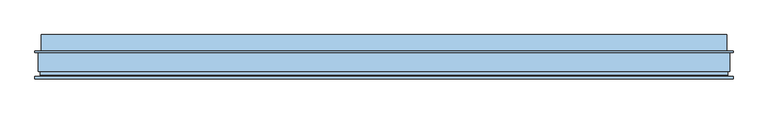
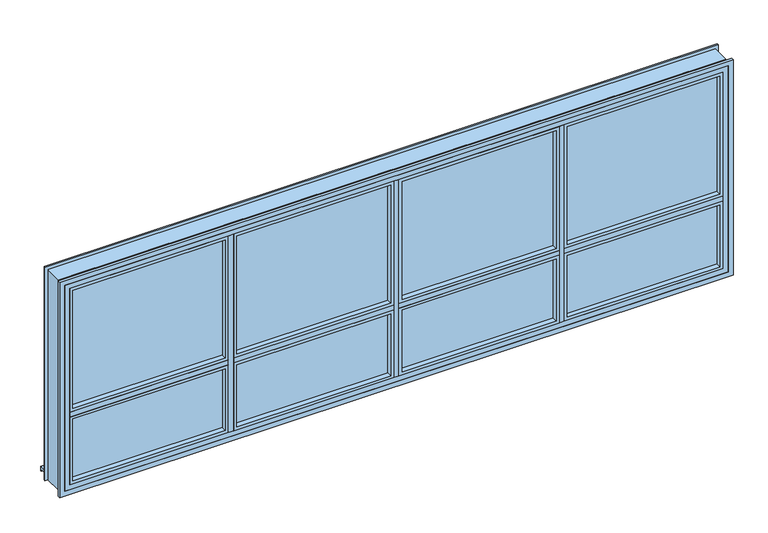
"""IFC4 building model written with IfcOpenShell, lengths in millimetres: window geometry, K-LINE ENSEMBLE COMPOSE NEUF KLT-8Z-4H2V : WD531_K-LINE ENSEMBLE COMPOSE NEUF KLT-8Z-4H2V."""

import ifcopenshell
import ifcopenshell.guid

model = None  # the IFC model being written
_history = None  # IfcOwnerHistory: only IFC2X3 demands one
_inside = {}  # id of a spatial element -> (the spatial element, [elements in it])
_under = {}  # id of a project, library or spatial element -> (it, [spatial elements below it])
_declared = {}  # id of a project -> (the project, [libraries it declares])
_typed = {}  # id of a type object -> (the type object, [elements of that type])
_made_of = {}  # id of a material, layer set ... -> (it, [elements and type objects made of it])


def new_model(schema):
    """Start an empty IFC model of exactly this schema.

    Asked for "IFC4X3", IfcOpenShell would pick the latest addendum, in which some entities
    have other attributes; the version numbers below select the first issue.
    IFC2X3 requires an IfcOwnerHistory on every rooted entity: one is made here for all.
    """
    global model, _history
    if schema == "IFC4X3":
        model = ifcopenshell.file(schema_version=(4, 3, 0, 0))
    else:
        model = ifcopenshell.file(schema=schema)
    _inside.clear()
    _under.clear()
    _declared.clear()
    _typed.clear()
    _made_of.clear()
    _history = None
    if model.schema == "IFC2X3":
        org = make("IfcOrganization", Name="unknown")
        user = make(
            "IfcPersonAndOrganization",
            ThePerson=make("IfcPerson", FamilyName="unknown"),
            TheOrganization=org,
        )
        app = make(
            "IfcApplication",
            ApplicationDeveloper=org,
            Version="unknown",
            ApplicationFullName="unknown",
            ApplicationIdentifier="unknown",
        )
        _history = make(
            "IfcOwnerHistory",
            OwningUser=user,
            OwningApplication=app,
            ChangeAction="ADDED",
            CreationDate=0,
        )
    return model


def make(cls, **values):
    """One entity of the class cls with the attributes given. An attribute that is None is left unset."""
    return model.create_entity(
        cls, **{name: value for name, value in values.items() if value is not None}
    )


def rooted(cls, **values):
    """An entity with a GlobalId (a new one), such as an element, a storey or a relation."""
    return make(cls, GlobalId=ifcopenshell.guid.new(), OwnerHistory=_history, **values)


def si_unit(unit_type, name, prefix=None):
    """IfcSIUnit, for example si_unit("LENGTHUNIT", "METRE", prefix="MILLI")."""
    return make("IfcSIUnit", UnitType=unit_type, Prefix=prefix, Name=name)


def assignment(units):
    """IfcUnitAssignment: the units of a project."""
    return None if units is None else make("IfcUnitAssignment", Units=units)


def point(xyz):
    """IfcCartesianPoint."""
    return None if xyz is None else make("IfcCartesianPoint", Coordinates=xyz)


def direction(xyz):
    """IfcDirection."""
    return None if xyz is None else make("IfcDirection", DirectionRatios=xyz)


def frame(location, z_axis=None, x_axis=None):
    """IfcAxis2Placement3D, a coordinate frame: its origin and axes. An axis left out is left unset."""
    return make(
        "IfcAxis2Placement3D",
        Location=point(location),
        Axis=direction(z_axis),
        RefDirection=direction(x_axis),
    )


def origin():
    """The frame at (0, 0, 0) with its axes left unset."""
    return frame((0.0, 0.0, 0.0))


def place(relative_to, where):
    """IfcLocalPlacement: puts the frame where relative to a parent placement (None: the world)."""
    return make(
        "IfcLocalPlacement", PlacementRelTo=relative_to, RelativePlacement=where
    )


def context(
    kind, dimensions, precision=None, world=None, true_north=None, identifier=None
):
    """IfcGeometricRepresentationContext, for example the 3D "Model" context."""
    return make(
        "IfcGeometricRepresentationContext",
        ContextIdentifier=identifier,
        ContextType=kind,
        CoordinateSpaceDimension=dimensions,
        Precision=precision,
        WorldCoordinateSystem=world,
        TrueNorth=true_north,
    )


def project(units=None, contexts=None):
    """IfcProject with its units and contexts."""
    return rooted(
        "IfcProject",
        Name="project",
        RepresentationContexts=contexts,
        UnitsInContext=assignment(units),
    )


def spatial(cls, under=None, at=None, **own):
    """A site, building, storey or space (cls), placed at a placement, below another one or the project."""
    s = rooted(cls, ObjectPlacement=at, **own)
    if under is not None:
        _under.setdefault(under.id(), (under, []))[1].append(s)
    return s


def polyline(points):
    """IfcPolyline through the points."""
    return make("IfcPolyline", Points=[point(p) for p in points])


def outline(outer, holes=None, kind="AREA"):
    """IfcArbitraryClosedProfileDef: a profile drawn as a closed curve; with holes, ...WithVoids."""
    if holes is None:
        return make("IfcArbitraryClosedProfileDef", ProfileType=kind, OuterCurve=outer)
    return make(
        "IfcArbitraryProfileDefWithVoids",
        ProfileType=kind,
        OuterCurve=outer,
        InnerCurves=holes,
    )


def extrude(swept, where, along, depth):
    """IfcExtrudedAreaSolid: the profile swept, set in the frame where, extruded along a direction by depth."""
    return make(
        "IfcExtrudedAreaSolid",
        SweptArea=swept,
        Position=where,
        ExtrudedDirection=direction(along),
        Depth=depth,
    )


def faces_of(points, faces, orient=None, outer=None):
    """IfcFace entities. A face is a list of loops; a loop is a list of indices into points, from 0.

    orient and outer hold one flag for each loop. By default every Orientation is true, the
    first loop of a face is its IfcFaceOuterBound and the others are IfcFaceBound.
    """
    made = []
    for i, loops in enumerate(faces):
        bounds = []
        for j, loop in enumerate(loops):
            is_outer = j == 0 if outer is None else outer[i][j]
            bounds.append(
                make(
                    "IfcFaceOuterBound" if is_outer else "IfcFaceBound",
                    Bound=make("IfcPolyLoop", Polygon=[points[k] for k in loop]),
                    Orientation=True if orient is None else orient[i][j],
                )
            )
        made.append(make("IfcFace", Bounds=bounds))
    return made


def faceted_brep(points, faces, orient=None, outer=None, voids=None):
    """IfcFacetedBrep: a solid bounded by flat faces; with voids (closed shells), ...WithVoids."""
    shared = [point(p) for p in points]
    hull = make("IfcClosedShell", CfsFaces=faces_of(shared, faces, orient, outer))
    if voids is None:
        return make("IfcFacetedBrep", Outer=hull)
    return make(
        "IfcFacetedBrepWithVoids",
        Outer=hull,
        Voids=[
            make(cls, CfsFaces=faces_of(shared, fs, o, b)) for cls, fs, o, b in voids
        ],
    )


def shape(context_of_items, identifier, shape_type, items):
    """IfcShapeRepresentation: the items that make up one representation, for example the "Body"."""
    return make(
        "IfcShapeRepresentation",
        ContextOfItems=context_of_items,
        RepresentationIdentifier=identifier,
        RepresentationType=shape_type,
        Items=items,
    )


def source(mapping_origin, context_of_items, identifier, shape_type, items):
    """IfcRepresentationMap: a shape defined once, which mapped items show again and again."""
    return make(
        "IfcRepresentationMap",
        MappingOrigin=mapping_origin,
        MappedRepresentation=shape(context_of_items, identifier, shape_type, items),
    )


def transform(
    local_origin,
    x_axis=None,
    y_axis=None,
    z_axis=None,
    scale=None,
    scale2=None,
    scale3=None,
    uniform=True,
):
    """IfcCartesianTransformationOperator3D, or its non-uniform kind. x_axis, y_axis, z_axis: its Axis1, 2, 3."""
    if uniform:
        return make(
            "IfcCartesianTransformationOperator3D",
            Axis1=direction(x_axis),
            Axis2=direction(y_axis),
            LocalOrigin=point(local_origin),
            Scale=scale,
            Axis3=direction(z_axis),
        )
    return make(
        "IfcCartesianTransformationOperator3DnonUniform",
        Axis1=direction(x_axis),
        Axis2=direction(y_axis),
        LocalOrigin=point(local_origin),
        Scale=scale,
        Axis3=direction(z_axis),
        Scale2=scale2,
        Scale3=scale3,
    )


def mapped(mapping_source, mapping_target):
    """IfcMappedItem: shows the shape of a source again, moved by a transform."""
    return make(
        "IfcMappedItem", MappingSource=mapping_source, MappingTarget=mapping_target
    )


def made_of(thing, what):
    """Note that an element or type object is made of a material, layer set ...; save() writes the relation."""
    if what is not None:
        _made_of.setdefault(what.id(), (what, []))[1].append(thing)
    return thing


def element(
    cls,
    number,
    at=None,
    inside=None,
    cuts=None,
    type_object=None,
    material=None,
    context=None,
    identifier="Body",
    shape_type=None,
    held_by="IfcProductDefinitionShape",
    body=None,
    shapes=None,
    **own,
):
    """One element of the class cls, such as IfcWall. Its Tag is "e" and its number.

    at: its placement. inside: the storey or other place that contains it. cuts: it is an
    opening in that element (IfcRelVoidsElement). A single representation is given by context,
    identifier, shape_type and body (its items); several are given by shapes. held_by: the class
    of the entity that holds the representations. save() writes the other relations.
    """
    e = rooted(cls, Tag="e%d" % number, ObjectPlacement=at, **own)
    if body is not None:
        shapes = [shape(context, identifier, shape_type, body)]
    if shapes is not None:
        e.Representation = make(held_by, Representations=shapes)
    if inside is not None:
        _inside.setdefault(inside.id(), (inside, []))[1].append(e)
    if cuts is not None:
        rooted(
            "IfcRelVoidsElement", RelatingBuildingElement=cuts, RelatedOpeningElement=e
        )
    if type_object is not None:
        _typed.setdefault(type_object.id(), (type_object, []))[1].append(e)
    return made_of(e, material)


def aggregate(whole, parts):
    """IfcRelAggregates: a whole, such as a stair, and the parts it consists of."""
    return rooted("IfcRelAggregates", RelatingObject=whole, RelatedObjects=parts)


def save(model, path):
    """Write the relations noted so far, then the file.

    IfcRelAggregates (storeys below a building ...), IfcRelContainedInSpatialStructure (elements
    in a storey), IfcRelDefinesByType, IfcRelAssociatesMaterial and IfcRelDeclares: one each for
    every whole, place, type object, material and project.
    """
    for whole, parts in _under.values():
        aggregate(whole, parts)
    for where, things in _inside.values():
        rooted(
            "IfcRelContainedInSpatialStructure",
            RelatedElements=things,
            RelatingStructure=where,
        )
    for kind, things in _typed.values():
        rooted("IfcRelDefinesByType", RelatedObjects=things, RelatingType=kind)
    for what, things in _made_of.values():
        rooted("IfcRelAssociatesMaterial", RelatedObjects=things, RelatingMaterial=what)
    for by, libraries in _declared.values():
        rooted("IfcRelDeclares", RelatingContext=by, RelatedDefinitions=libraries)
    model.write(path)


def window_16f5b6b2(model_context):
    return source(origin(), model_context, "Body", "SolidModel", [
        extrude(outline(polyline([(-18.0, -155.0), (-18.0, -179.0), (-882.0, -179.0), (-882.0, -155.0), (-18.0, -155.0)])), frame((0.0, 0.0, 850.5), z_axis=(0.0, 0.0, 1.0), x_axis=(1.0, 0.0, 0.0)), (0.0, 0.0, 1.0), 381.5),
        extrude(outline(polyline([(1236.0, -14.0), (1236.0, -886.0), (846.5, -886.0), (846.5, -14.0), (1236.0, -14.0)]), holes=[polyline([(863.5, -31.0), (863.5, -869.0), (1219.0, -869.0), (1219.0, -31.0), (863.5, -31.0)])]), frame((0.0, -207.5, 0.0), z_axis=(0.0, 1.0, 0.0), x_axis=(0.0, 0.0, 1.0)), (0.0, 0.0, 1.0), 28.5),
        extrude(outline(polyline([(-18.0, -155.0), (-18.0, -179.0), (-882.0, -179.0), (-882.0, -155.0), (-18.0, -155.0)])), frame((0.0, 0.0, 1268.0), z_axis=(0.0, 0.0, 1.0), x_axis=(1.0, 0.0, 0.0)), (0.0, 0.0, 1.0), 705.0),
        extrude(outline(polyline([(1977.0, -14.0), (1977.0, -886.0), (1264.0, -886.0), (1264.0, -14.0), (1977.0, -14.0)]), holes=[polyline([(1281.0, -31.0), (1281.0, -869.0), (1960.0, -869.0), (1960.0, -31.0), (1281.0, -31.0)])]), frame((0.0, -207.5, 0.0), z_axis=(0.0, 1.0, 0.0), x_axis=(0.0, 0.0, 1.0)), (0.0, 0.0, 1.0), 28.5),
        extrude(outline(polyline([(-188.500001, 1241.0), (-188.500001, 1259.0), (-155.0, 1259.0), (-155.0, 1284.0), (-147.5, 1284.0), (-147.5, 1216.0), (-155.000001, 1216.0), (-155.000001, 1241.0), (-188.500001, 1241.0)])), frame((-866.0, 0.0, 0.0), z_axis=(1.0, 0.0, 0.0), x_axis=(0.0, 1.0, 0.0)), (0.0, 0.0, 1.0), 832.0),
        extrude(outline(polyline([(-14.0, -207.5), (-886.0, -207.5), (-886.0, -188.500001), (-14.0, -188.500001), (-14.0, -207.5)])), frame((0.0, 0.0, 1236.0), z_axis=(0.0, 0.0, 1.0), x_axis=(1.0, 0.0, 0.0)), (0.0, 0.0, 1.0), 28.0),
        extrude(outline(polyline([(-891.0, -155.0), (-891.0, -188.5), (-909.0, -188.5), (-909.0, -155.0), (-934.0, -155.0), (-934.0, -147.5), (-866.0, -147.5), (-866.0, -155.0), (-891.0, -155.0)])), frame((0.0, 0.0, 866.5), z_axis=(0.0, 0.0, 1.0), x_axis=(1.0, 0.0, 0.0)), (0.0, 0.0, 1.0), 1090.5),
        extrude(outline(polyline([(-914.0, -207.5), (-914.0, -188.5), (-886.0, -188.5), (-886.0, -207.5), (-914.0, -207.5)])), frame((0.0, 0.0, 846.5), z_axis=(0.0, 0.0, 1.0), x_axis=(1.0, 0.0, 0.0)), (0.0, 0.0, 1.0), 1130.5),
        extrude(outline(polyline([(882.0, -155.0), (882.0, -179.0), (18.0, -179.0), (18.0, -155.0), (882.0, -155.0)])), frame((0.0, 0.0, 850.5), z_axis=(0.0, 0.0, 1.0), x_axis=(1.0, 0.0, 0.0)), (0.0, 0.0, 1.0), 381.5),
        extrude(outline(polyline([(1236.0, 886.0), (1236.0, 14.0), (846.5, 14.0), (846.5, 886.0), (1236.0, 886.0)]), holes=[polyline([(863.5, 869.0), (863.5, 31.0), (1219.0, 31.0), (1219.0, 869.0), (863.5, 869.0)])]), frame((0.0, -207.5, 0.0), z_axis=(0.0, 1.0, 0.0), x_axis=(0.0, 0.0, 1.0)), (0.0, 0.0, 1.0), 28.5),
        extrude(outline(polyline([(882.0, -155.0), (882.0, -179.0), (18.0, -179.0), (18.0, -155.0), (882.0, -155.0)])), frame((0.0, 0.0, 1268.0), z_axis=(0.0, 0.0, 1.0), x_axis=(1.0, 0.0, 0.0)), (0.0, 0.0, 1.0), 705.0),
        extrude(outline(polyline([(1977.0, 886.0), (1977.0, 14.0), (1264.0, 14.0), (1264.0, 886.0), (1977.0, 886.0)]), holes=[polyline([(1281.0, 869.0), (1281.0, 31.0), (1960.0, 31.0), (1960.0, 869.0), (1281.0, 869.0)])]), frame((0.0, -207.5, 0.0), z_axis=(0.0, 1.0, 0.0), x_axis=(0.0, 0.0, 1.0)), (0.0, 0.0, 1.0), 28.5),
        extrude(outline(polyline([(-188.500001, 1241.0), (-188.500001, 1259.0), (-155.0, 1259.0), (-155.0, 1284.0), (-147.5, 1284.0), (-147.5, 1216.0), (-155.000001, 1216.0), (-155.000001, 1241.0), (-188.500001, 1241.0)])), frame((34.0, 0.0, 0.0), z_axis=(1.0, 0.0, 0.0), x_axis=(0.0, 1.0, 0.0)), (0.0, 0.0, 1.0), 832.0),
        extrude(outline(polyline([(886.0, -207.5), (14.0, -207.5), (14.0, -188.500001), (886.0, -188.500001), (886.0, -207.5)])), frame((0.0, 0.0, 1236.0), z_axis=(0.0, 0.0, 1.0), x_axis=(1.0, 0.0, 0.0)), (0.0, 0.0, 1.0), 28.0),
        extrude(outline(polyline([(9.0, -155.0), (9.0, -188.5), (-9.0, -188.5), (-9.0, -155.0), (-34.0, -155.0), (-34.0, -147.5), (34.0, -147.5), (34.0, -155.0), (9.0, -155.0)])), frame((0.0, 0.0, 866.5), z_axis=(0.0, 0.0, 1.0), x_axis=(1.0, 0.0, 0.0)), (0.0, 0.0, 1.0), 1090.5),
        extrude(outline(polyline([(-14.0, -207.5), (-14.0, -188.5), (14.0, -188.5), (14.0, -207.5), (-14.0, -207.5)])), frame((0.0, 0.0, 846.5), z_axis=(0.0, 0.0, 1.0), x_axis=(1.0, 0.0, 0.0)), (0.0, 0.0, 1.0), 1130.5),
        extrude(outline(polyline([(1773.0, -155.0), (1773.0, -179.0), (918.0, -179.0), (918.0, -155.0), (1773.0, -155.0)])), frame((0.0, 0.0, 850.5), z_axis=(0.0, 0.0, 1.0), x_axis=(1.0, 0.0, 0.0)), (0.0, 0.0, 1.0), 381.5),
        extrude(outline(polyline([(1236.0, 1777.0), (1236.0, 914.0), (846.5, 914.0), (846.5, 1777.0), (1236.0, 1777.0)]), holes=[polyline([(863.5, 1760.0), (863.5, 931.0), (1219.0, 931.0), (1219.0, 1760.0), (863.5, 1760.0)])]), frame((0.0, -207.5, 0.0), z_axis=(0.0, 1.0, 0.0), x_axis=(0.0, 0.0, 1.0)), (0.0, 0.0, 1.0), 28.5),
        extrude(outline(polyline([(-918.0, -155.0), (-918.0, -179.0), (-1773.0, -179.0), (-1773.0, -155.0), (-918.0, -155.0)])), frame((0.0, 0.0, 850.5), z_axis=(0.0, 0.0, 1.0), x_axis=(1.0, 0.0, 0.0)), (0.0, 0.0, 1.0), 381.5),
        extrude(outline(polyline([(1236.0, -914.0), (1236.0, -1777.0), (846.5, -1777.0), (846.5, -914.0), (1236.0, -914.0)]), holes=[polyline([(863.5, -931.0), (863.5, -1760.0), (1219.0, -1760.0), (1219.0, -931.0), (863.5, -931.0)])]), frame((0.0, -207.5, 0.0), z_axis=(0.0, 1.0, 0.0), x_axis=(0.0, 0.0, 1.0)), (0.0, 0.0, 1.0), 28.5),
        extrude(outline(polyline([(-188.500001, 1241.0), (-188.500001, 1259.0), (-155.0, 1259.0), (-155.0, 1284.0), (-147.5, 1284.0), (-147.5, 1216.0), (-155.000001, 1216.0), (-155.000001, 1241.0), (-188.500001, 1241.0)])), frame((-1757.0, 0.0, 0.0), z_axis=(1.0, 0.0, 0.0), x_axis=(0.0, 1.0, 0.0)), (0.0, 0.0, 1.0), 823.0),
        extrude(outline(polyline([(-914.0, -207.5), (-1777.0, -207.5), (-1777.0, -188.500001), (-914.0, -188.500001), (-914.0, -207.5)])), frame((0.0, 0.0, 1236.0), z_axis=(0.0, 0.0, 1.0), x_axis=(1.0, 0.0, 0.0)), (0.0, 0.0, 1.0), 28.0),
        extrude(outline(polyline([(-188.500001, 1241.0), (-188.500001, 1259.0), (-155.0, 1259.0), (-155.0, 1284.0), (-147.5, 1284.0), (-147.5, 1216.0), (-155.000001, 1216.0), (-155.000001, 1241.0), (-188.500001, 1241.0)])), frame((934.0, 0.0, 0.0), z_axis=(1.0, 0.0, 0.0), x_axis=(0.0, 1.0, 0.0)), (0.0, 0.0, 1.0), 823.0),
        extrude(outline(polyline([(1777.0, -207.5), (914.0, -207.5), (914.0, -188.500001), (1777.0, -188.500001), (1777.0, -207.5)])), frame((0.0, 0.0, 1236.0), z_axis=(0.0, 0.0, 1.0), x_axis=(1.0, 0.0, 0.0)), (0.0, 0.0, 1.0), 28.0),
        extrude(outline(polyline([(1773.0, -155.0), (1773.0, -179.0), (918.0, -179.0), (918.0, -155.0), (1773.0, -155.0)])), frame((0.0, 0.0, 1268.0), z_axis=(0.0, 0.0, 1.0), x_axis=(1.0, 0.0, 0.0)), (0.0, 0.0, 1.0), 705.0),
        extrude(outline(polyline([(1977.0, 1777.0), (1977.0, 914.0), (1264.0, 914.0), (1264.0, 1777.0), (1977.0, 1777.0)]), holes=[polyline([(1281.0, 1760.0), (1281.0, 931.0), (1960.0, 931.0), (1960.0, 1760.0), (1281.0, 1760.0)])]), frame((0.0, -207.5, 0.0), z_axis=(0.0, 1.0, 0.0), x_axis=(0.0, 0.0, 1.0)), (0.0, 0.0, 1.0), 28.5),
        extrude(outline(polyline([(-918.0, -155.0), (-918.0, -179.0), (-1773.0, -179.0), (-1773.0, -155.0), (-918.0, -155.0)])), frame((0.0, 0.0, 1268.0), z_axis=(0.0, 0.0, 1.0), x_axis=(1.0, 0.0, 0.0)), (0.0, 0.0, 1.0), 705.0),
        extrude(outline(polyline([(1977.0, -914.0), (1977.0, -1777.0), (1264.0, -1777.0), (1264.0, -914.0), (1977.0, -914.0)]), holes=[polyline([(1281.0, -931.0), (1281.0, -1760.0), (1960.0, -1760.0), (1960.0, -931.0), (1281.0, -931.0)])]), frame((0.0, -207.5, 0.0), z_axis=(0.0, 1.0, 0.0), x_axis=(0.0, 0.0, 1.0)), (0.0, 0.0, 1.0), 28.5),
        extrude(outline(polyline([(909.0, -155.0), (909.0, -188.5), (891.0, -188.5), (891.0, -155.0), (866.0, -155.0), (866.0, -147.5), (934.0, -147.5), (934.0, -155.0), (909.0, -155.0)])), frame((0.0, 0.0, 866.5), z_axis=(0.0, 0.0, 1.0), x_axis=(1.0, 0.0, 0.0)), (0.0, 0.0, 1.0), 1090.5),
        extrude(outline(polyline([(886.0, -207.5), (886.0, -188.5), (914.0, -188.5), (914.0, -207.5), (886.0, -207.5)])), frame((0.0, 0.0, 846.5), z_axis=(0.0, 0.0, 1.0), x_axis=(1.0, 0.0, 0.0)), (0.0, 0.0, 1.0), 1130.5),
        extrude(outline(polyline([(2032.0, 1832.0), (2032.0, -1832.0), (791.5, -1832.0), (791.5, 1832.0), (2032.0, 1832.0)]), holes=[polyline([(818.4999998, 1805.0000002), (818.4999998, -1805.0000002), (2005.0000002, -1805.0000002), (2005.0000002, 1805.0000002), (818.4999998, 1805.0000002)])]), frame((0.0, -207.5, 0.0), z_axis=(0.0, 1.0, 0.0), x_axis=(0.0, 0.0, 1.0)), (0.0, 0.0, 1.0), 12.5),
        extrude(outline(polyline([(2005.0000002, 1805.0000002), (2005.0000002, -1805.0000002), (818.4999998, -1805.0000002), (818.4999998, 1805.0000002), (2005.0000002, 1805.0000002)]), holes=[polyline([(846.5, 1777.0), (846.5, -1777.0), (1977.0, -1777.0), (1977.0, 1777.0), (846.5, 1777.0)])]), frame((0.0, -207.5, 0.0), z_axis=(0.0, 1.0, 0.0), x_axis=(0.0, 0.0, 1.0)), (0.0, 0.0, 1.0), 19.0),
        faceted_brep([(1756.999999, -154.9965859, 1956.999999), (1756.999999, -147.4965859, 1956.999999), (1756.999999, -147.4965859, 866.500001), (1756.999999, -154.9965859, 866.500001), (1805.0000002, -147.4965859, 818.4999998), (-1805.0000002, -147.4965859, 818.4999998), (-1805.0000002, -147.4965859, 2005.0000002), (1805.0000002, -147.4965859, 2005.0000002), (-1756.999999, -147.4965859, 1956.999999), (-1756.999999, -147.4965859, 866.500001), (-1756.999999, -154.9965859, 866.500001), (1782.0, -154.9965859, 1982.0), (-1782.0, -154.9965859, 1982.0), (-1782.0, -154.9965859, 841.5), (1782.0, -154.9965859, 841.5), (-1756.999999, -154.9965859, 1956.999999), (1782.0, -188.5, 1982.0), (1782.0, -188.5, 841.5), (-1782.0, -188.5, 841.5), (1805.0000002, -188.5, 2005.0000002), (-1805.0000002, -188.5, 2005.0000002), (-1805.0000002, -188.5, 818.4999998), (1805.0000002, -188.5, 818.4999998), (-1782.0, -188.5, 1982.0)], [[[0, 1, 2, 3]], [[4, 5, 6, 7], [1, 8, 9, 2]], [[3, 2, 9, 10]], [[11, 12, 13, 14], [3, 10, 15, 0]], [[16, 11, 14, 17]], [[17, 14, 13, 18]], [[19, 20, 21, 22], [17, 18, 23, 16]], [[7, 19, 22, 4]], [[4, 22, 21, 5]], [[10, 9, 8, 15]], [[18, 13, 12, 23]], [[5, 21, 20, 6]], [[15, 8, 1, 0]], [[23, 12, 11, 16]], [[6, 20, 19, 7]]]),
        faceted_brep([(-1815.0, -68.0, 805.0), (-1832.0, -68.0, 805.0), (-1832.0, -60.0, 805.0), (-1800.0, -60.0, 805.0), (-1800.0, -147.4965859, 805.0), (-1805.0, -147.4965859, 805.0), (-1805.0, -166.4965859, 805.0), (-1815.0, -166.4965859, 805.0), (-1815.0, -68.0, 2015.0), (1815.0, -68.0, 2015.0), (1815.0, -68.0, 805.0), (1832.0, -68.0, 805.0), (1832.0, -68.0, 2032.0), (-1832.0, -68.0, 2032.0), (-1832.0, -60.0, 2032.0), (1832.0, -60.0, 2032.0), (1832.0, -60.0, 805.0), (1800.0, -60.0, 805.0), (1800.0, -60.0, 2000.0), (-1800.0, -60.0, 2000.0), (-1800.0, -147.4965859, 2000.0), (1800.0, -147.4965859, 2000.0), (1800.0, -147.4965859, 805.0), (1805.0, -147.4965859, 805.0), (1805.0, -147.4965859, 2005.0), (-1805.0, -147.4965859, 2005.0), (-1805.0, -166.4965859, 2005.0), (1805.0, -166.4965859, 2005.0), (1805.0, -166.4965859, 805.0), (1815.0, -166.4965859, 805.0), (1815.0, -166.4965859, 2015.0), (-1815.0, -166.4965859, 2015.0)], [[[0, 1, 2, 3, 4, 5, 6, 7]], [[1, 0, 8, 9, 10, 11, 12, 13]], [[2, 1, 13, 14]], [[3, 2, 14, 15, 16, 17, 18, 19]], [[5, 4, 20, 21, 22, 23, 24, 25]], [[6, 5, 25, 26]], [[7, 6, 26, 27, 28, 29, 30, 31]], [[0, 7, 31, 8]], [[15, 12, 11, 16]], [[10, 29, 28, 23, 22, 17, 16, 11]], [[27, 24, 23, 28]], [[9, 30, 29, 10]], [[14, 13, 12, 15]], [[26, 25, 24, 27]], [[8, 31, 30, 9]], [[4, 3, 19, 20]], [[21, 18, 17, 22]], [[20, 19, 18, 21]]]),
        extrude(outline(polyline([(-147.4965859, 825.311129), (25.8038196, 819.2593455), (25.8038196, 794.3604516), (21.4038196, 794.3604516), (21.4038196, 805.0000004), (-161.2965876, 805.0000004), (-161.2965876, 818.5), (-147.4965859, 818.5), (-147.4965859, 825.311129)])), frame((-1800.0, 0.0, 0.0), z_axis=(1.0, 0.0, 0.0), x_axis=(0.0, 1.0, 0.0)), (0.0, 0.0, 1.0), 3600.0),
    ])


if __name__ == "__main__":
    model = new_model("IFC4")
    model_context = context("Model", 3, world=origin())
    ifc_project = project(units=[si_unit("LENGTHUNIT", "METRE", prefix="MILLI")], contexts=[model_context])
    site = spatial("IfcSite", under=ifc_project)
    building = spatial("IfcBuilding", under=site)
    placement = place(None, origin())
    window_shape = window_16f5b6b2(model_context)
    element("IfcWindow", 1, ObjectType="K-LINE ENSEMBLE COMPOSE NEUF KLT-8Z-4H2V : WD531_K-LINE ENSEMBLE COMPOSE NEUF KLT-8Z-4H2V", at=placement, inside=building, context=model_context, shape_type="MappedRepresentation", body=[
        mapped(window_shape, transform((0.0, 0.0, 0.0), x_axis=(1.0, 0.0, 0.0), y_axis=(0.0, 1.0, 0.0), z_axis=(0.0, 0.0, 1.0))),
    ])
    save(model, "model.ifc")

# Revit data of these elements
# Project information
#   Building Name = "MAIN GATE SECURITY BUILDING"
#   Project Status = "Project Status"
#   Client Name = "현대엔지니어링"
#   Project Address = "서울시 종로구 율곡로 75(계동)"
#   Project Name = "Therma Visayas Energy Project"
#   Project Number = "-"
# Type "K-LINE ENSEMBLE COMPOSE NEUF KLT-8Z-4H2V : WD531_K-LINE ENSEMBLE COMPOSE NEUF KLT-8Z-4H2V"
#   Type Mark = "AW"
#   Vitrage secondaire = ""
#   Vitrage principal = ""
#   URL = "https://pro.k-line.fr/bandes-ensembles-composes-kl-t.aspx"
#   Type de pose = "ITI"
#   Transmission lumineuse TLw = "67%"
#   SAV = "https://sav.k-line.fr/"
#   Product data url = "https://www.bimobject.com/k-line/product/klt-8zec2h4v"
#   Outil de thermo-luminosité = "http://www.pro.k-line.fr/calculateur-presentation.aspx"
#   Occultation = "Non"
#   Numéro de série = "K.........."
#   Keynote = "08520"
#   Neuf / Réno / Multi support = "Neuf"
#   Mortaise et grille d'entrée d'air = ""
#   Model = "KL-T Châssis Ensemble composé 8 Zones"
#   Matériaux = "Aluminium et verre"
#   Information renfort d'inertie = "Les renforts intérieurs ne sont compatible avec des ouvrants que sur des profils de 200mm de largeur"
#   Garanties = "https://pro.k-line.fr/pdf/attestations/Garanties_Legales_KLINE.pdf"
#   Famille de produit = "KL-City"
#   Manufacturer = "K.LINE"
#   Entretien = "https://pro.k-line.fr/pdf/ficheproduit/laq_fiche_entretien.pdf"
#   Entreprise de pose = ""
#   Doublages disponibles = "80,100,110,120,130,140,160,180 et 200 mm"
#   Description = "Fenêtre Alu"
#   Analytic Construction = "<Aucun>"
#   Composition analytique de base = "Châssis 1250x1480 - Vitrage 4/WE Argon 16/TBE 4 - Finition Black"
#   Classement AEV = "A*4 E*7B V*A3"
#   Classe COV = "A+"
#   Avis technique = "https://pro.k-line.fr/attestations-avis-technique.aspx"
#   Affaiblissement acoustique R(A,tr) = "30dB"
#   Val décal appui = 100 mm
#   Transmission thermique Uw = 1.4000 W/(m²·K)
#   Surface = 4.32 m²
#   Profondeur symbole d'ouverture = 150 mm
#   Position doublage = 0 mm
#   Lg traverse 4 = 909 mm
#   Lg traverse 3 = 918 mm
#   Lg traverse 2 = 918 mm
#   Lg traverse 1 = 909 mm
#   Largeur zone 4 = 900 mm
#   Largeur zone 3 = 900 mm
#   Largeur zone 2 = 900 mm
#   Largeur zone 1 = 900 mm
#   Largeur ouvrant 4 = 839 mm
#   Largeur ouvrant 3 = 848 mm
#   Largeur ouvrant 2 = 848 mm
#   Largeur ouvrant 1 = 839 mm
#   Rough Width [instance default] = 3600 mm
#   Largeur Traverse intermédiaire : 68,85,100,150,175 et 200 = 68 mm
#   Largeur Montant intermédiaire : 68,85,100,150,175 et 200 = 68 mm
#   Hauteur zone 5 = 750 mm
#   Hauteur zone 1 = 450 mm
#   Hauteur ouvrant 4/5/6 = 689 mm
#   Hauteur ouvrant 1/2/3 = 365.5 mm
#   Hauteur de poignée = 318 mm
#   Rough Height [instance default] = 1200 mm
#   Height = 1200 mm
#   Hauteur de l'appui par défaut = 800 mm
#   H profil = 1090.5 mm
#   Width = 3600 mm
#   Facteur solaire ScW (Hiver) = 0.53
#   Décalage appui = 180 mm
#   Décal appui = 40 mm
#   Doublage + ratrapage = 140 mm
#   Doublage = 140 mm
#   Centre zone 5/6/7/8 = 344.5 mm
#   Centre zone 1/2/3/4 = 182.75 mm
#   Centre Ouvrant 4/8 = 419.5 mm
#   Centre Ouvrant 3/7 = 450 mm
#   Centre Ouvrant 2/6 = 450 mm
#   Centre Ouvrant 1/5 = 419.5 mm
#   Angle symbole d'ouverture = 15.00°
#   Symbole d'ouverture = yes
#   Renfort saillant Intérieur = no
#   Renfort saillant Extérieur = no
#   Renfort Int saillant de 67.5 = no
#   Renfort Int saillant de 107.5 = yes
#   Renfort Ext saillant de 67.5 = no
#   Renfort Ext saillant de 107.5 = yes
#   Rattrapage doublage = no
#   Option appui sans aile intérieure = no
#   Finition Métal = yes
#   Finition Black = no
#   Rattrapage avec aile = no
#   Appui Non-Déporté = no
#   Appui Déporté = yes
#   Vitrage = Verre
#   Type d'ouvrant zone 8 = element 2302654
#   Type d'ouvrant zone 7 = element 2302654
#   Type d'ouvrant zone 6 = element 2302654
#   Type d'ouvrant zone 5 = element 2302654
#   Type d'ouvrant zone 4 = element 2302654
#   Type d'ouvrant zone 3 = element 2302654
#   Type d'ouvrant zone 2 = element 2302654
#   Type d'ouvrant zone 1 = element 2302654
#   Couleur panneau opaque Int = K.Line Intemporel Blanc satiné (9016 S) - KQ
#   Couleur panneau opaque Ext = K.Line Tendance Grège (9007 T) - RQ
#   Couleur châssis Int = K.Line Intemporel Blanc satiné (9016 S) - KQ
#   Couleur châssis Ext = K.Line Tendance Grège (9007 T) - RQ
#   Couleur Accessoire Int = K.Line Accessoire Blanc - KQ
#   Wall Closure = (empty or 0)
# Element 1 (IfcWindow, "K-LINE ENSEMBLE COMPOSE NEUF KLT-8Z-4H2V : WD531_K-LINE ENSEMBLE COMPOSE NEUF KLT-8Z-4H2V")
#   Materials on its faces: "K.Line Intemporel Blanc satiné (9016 S) - KQ", "K.Line Tendance Grège (9007 T) - RQ", "Verre"
# Materials
#   "Verre": class "Verre", colour RGB 92 99 177, transparency 0.7, Description = "AL. WINDOW(TYP.)", Cost = 0
#   "K.Line Intemporel Blanc satiné (9016 S) - KQ": class "Metal", colour RGB 247 246 246, transparency 0, Description = "Aluminum 6061", Cost = 0
#   "K.Line Tendance Grège (9007 T) - RQ": class "Metal", colour RGB 135 133 129, transparency 0, Description = "Aluminum 6061", Cost = 0
#   "K.Line Accessoire Blanc - KQ": class "Metal", colour RGB 247 246 246, transparency 0, Description = "Aluminum 6061", Cost = 0
